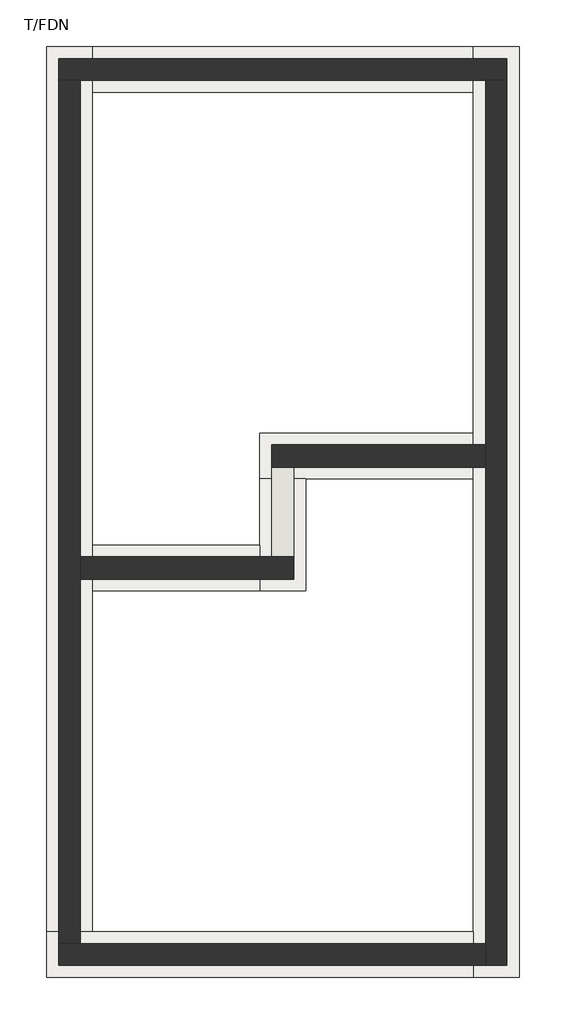
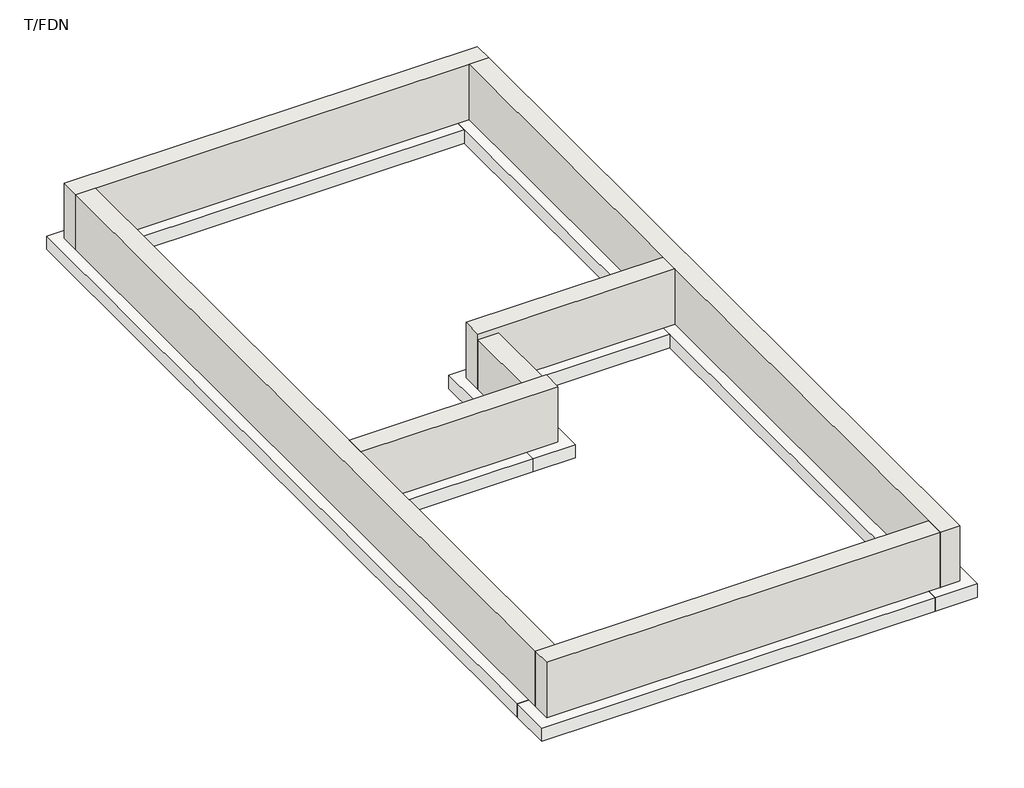
# One storey: 7 footings, 7 walls.
"""IFC4 building model written with IfcOpenShell, lengths in millimetres."""

from ifc_helpers import new_model, si_unit, frame, origin, place, context, project, spatial, polyline, outline, extrude, faceted_brep, element, save

model = new_model("IFC4")

# Units and contexts
model_context = context("Model", 3, world=origin())
ifc_project = project(units=[si_unit("LENGTHUNIT", "METRE", prefix="MILLI")], contexts=[model_context])

# Site, building, storey
site = spatial("IfcSite", under=ifc_project)
building = spatial("IfcBuilding", under=site)
storey = spatial("IfcBuildingStorey", under=building, Name="T/FDN", Elevation=-1250.0)

# Footings
placement = place(None, origin())
element("IfcFooting", 1, ObjectType="Bearing Footing - 900 x 300", at=placement, inside=storey, context=model_context, shape_type="Brep", body=[
    faceted_brep([(8141.5, 241.5, -1250.0), (8141.5, -658.5, -1250.0), (8141.5, -7350.0, -1250.0), (8141.5, -8250.0, -1250.0), (8141.5, -17141.5, -1250.0), (8141.5, -18041.5, -1250.0), (9041.5, -18041.5, -1250.0), (9041.5, 241.5, -1250.0), (9041.5, 241.5, -1550.0), (9041.5, -18041.5, -1550.0), (8141.5, 241.5, -1550.0), (8141.5, -18041.5, -1550.0), (8141.5, -17141.5, -1550.0), (8141.5, -8250.0, -1550.0), (8141.5, -7350.0, -1550.0), (8141.5, -658.5, -1550.0)], [[[0, 1, 2, 3, 4, 5, 6, 7]], [[8, 7, 6, 9]], [[10, 8, 9, 11, 12, 13, 14, 15]], [[0, 10, 15, 14, 13, 12, 11, 5, 4, 3, 2, 1]], [[6, 5, 11, 9]], [[0, 7, 8, 10]]]),
])
element("IfcFooting", 2, ObjectType="Bearing Footing - 900 x 300", at=placement, inside=storey, context=model_context, shape_type="Brep", body=[
    faceted_brep([(-241.5, -17141.5, -1250.0), (-241.5, -18041.5, -1250.0), (8141.5, -18041.5, -1250.0), (8141.5, -17141.5, -1250.0), (658.5, -17141.5, -1250.0), (-241.5, -18041.5, -1550.0), (8141.5, -18041.5, -1550.0), (-241.5, -17141.5, -1550.0), (658.5, -17141.5, -1550.0), (8141.5, -17141.5, -1550.0)], [[[0, 1, 2, 3, 4]], [[1, 5, 6, 2]], [[5, 7, 8, 9, 6]], [[7, 0, 4, 3, 9, 8]], [[3, 2, 6, 9]], [[1, 0, 7, 5]]]),
])
element("IfcFooting", 3, ObjectType="Bearing Footing - 900 x 300", at=placement, inside=storey, context=model_context, shape_type="Brep", body=[
    faceted_brep([(658.5, 241.5, -1250.0), (-241.5, 241.5, -1250.0), (-241.5, -17141.5, -1250.0), (658.5, -17141.5, -1250.0), (658.5, -10450.0, -1250.0), (658.5, -9550.0, -1250.0), (658.5, -658.5, -1250.0), (-241.5, 241.5, -1550.0), (-241.5, -17141.5, -1550.0), (658.5, 241.5, -1550.0), (658.5, -658.5, -1550.0), (658.5, -9550.0, -1550.0), (658.5, -10450.0, -1550.0), (658.5, -17141.5, -1550.0)], [[[0, 1, 2, 3, 4, 5, 6]], [[1, 7, 8, 2]], [[7, 9, 10, 11, 12, 13, 8]], [[9, 0, 6, 5, 4, 3, 13, 12, 11, 10]], [[3, 2, 8, 13]], [[1, 0, 9, 7]]]),
])
element("IfcFooting", 4, ObjectType="Bearing Footing - 900 x 300", at=placement, inside=storey, context=model_context, shape_type="SweptSolid", body=[
    extrude(outline(polyline([(8141.5, 241.5), (8141.5, -658.5), (658.5, -658.5), (658.5, 241.5), (8141.5, 241.5)])), frame((0.0, 0.0, -1550.0), z_axis=(0.0, 0.0, 1.0), x_axis=(1.0, 0.0, 0.0)), (0.0, 0.0, 1.0), 300.0),
])
element("IfcFooting", 5, ObjectType="Bearing Footing - 900 x 300", at=placement, inside=storey, context=model_context, shape_type="Brep", body=[
    faceted_brep([(8141.5, -7350.0, -1250.0), (3950.0, -7350.0, -1250.0), (3950.0, -8250.0, -1250.0), (4850.0, -8250.0, -1250.0), (8141.5, -8250.0, -1250.0), (8141.5, -8250.0, -1550.0), (3950.0, -8250.0, -1550.0), (4850.0, -8250.0, -1550.0), (8141.5, -7350.0, -1550.0), (3950.0, -7350.0, -1550.0)], [[[0, 1, 2, 3, 4]], [[5, 4, 3, 2, 6, 7]], [[8, 5, 7, 6, 9]], [[0, 8, 9, 1]], [[0, 4, 5, 8]], [[2, 1, 9, 6]]]),
])
element("IfcFooting", 6, ObjectType="Bearing Footing - 900 x 300", at=placement, inside=storey, context=model_context, shape_type="Brep", body=[
    faceted_brep([(3950.0, -10450.0, -1250.0), (4850.0, -10450.0, -1250.0), (4850.0, -8250.0, -1250.0), (3950.0, -8250.0, -1250.0), (3950.0, -9550.0, -1250.0), (3950.0, -10450.0, -1550.0), (3950.0, -8250.0, -1550.0), (3950.0, -9550.0, -1550.0), (4850.0, -10450.0, -1550.0), (4850.0, -8250.0, -1550.0)], [[[0, 1, 2, 3, 4]], [[5, 0, 4, 3, 6, 7]], [[8, 5, 7, 6, 9]], [[1, 8, 9, 2]], [[1, 0, 5, 8]], [[3, 2, 9, 6]]]),
])
element("IfcFooting", 7, ObjectType="Bearing Footing - 900 x 300", at=placement, inside=storey, context=model_context, shape_type="SweptSolid", body=[
    extrude(outline(polyline([(658.5, -10450.0), (658.5, -9550.0), (3950.0, -9550.0), (3950.0, -10450.0), (658.5, -10450.0)])), frame((0.0, 0.0, -1550.0), z_axis=(0.0, 0.0, 1.0), x_axis=(1.0, 0.0, 0.0)), (0.0, 0.0, 1.0), 300.0),
])

# Walls
element("IfcWall", 8, ObjectType="Foundation - Concrete (417mm)", at=placement, inside=storey, context=model_context, shape_type="Brep", body=[
    faceted_brep([(0.0, -417.0, -1250.0), (417.0, -417.0, -1250.0), (8383.0, -417.0, -1250.0), (8800.0, -417.0, -1250.0), (8800.0, -417.0, 0.0), (8383.0, -417.0, 0.0), (417.0, -417.0, 0.0), (0.0, -417.0, 0.0), (0.0, 0.0, -1250.0), (0.0, 0.0, 0.0), (8800.0, 0.0, 0.0), (8800.0, 0.0, -1250.0)], [[[0, 1, 2, 3, 4, 5, 6, 7]], [[8, 9, 10, 11]], [[3, 2, 1, 0, 8, 11]], [[7, 6, 5, 4, 10, 9]], [[4, 3, 11, 10]], [[0, 7, 9, 8]]]),
])
element("IfcWall", 9, ObjectType="Foundation - Concrete (417mm)", at=placement, inside=storey, context=model_context, shape_type="Brep", body=[
    faceted_brep([(8383.0, -417.0, -1250.0), (8383.0, -7582.5, -1250.0), (8383.0, -8017.5, -1250.0), (8383.0, -17383.0, -1250.0), (8383.0, -17800.0, -1250.0), (8383.0, -17800.0, 0.0), (8383.0, -17383.0, 0.0), (8383.0, -8017.5, 0.0), (8383.0, -7582.5, 0.0), (8383.0, -417.0, 0.0), (8800.0, -417.0, -1250.0), (8800.0, -417.0, 0.0), (8800.0, -17800.0, 0.0), (8800.0, -17800.0, -1250.0)], [[[0, 1, 2, 3, 4, 5, 6, 7, 8, 9]], [[10, 11, 12, 13]], [[4, 3, 2, 1, 0, 10, 13]], [[9, 8, 7, 6, 5, 12, 11]], [[0, 9, 11, 10]], [[5, 4, 13, 12]]]),
])
element("IfcWall", 10, ObjectType="Foundation - Concrete (417mm)", at=placement, inside=storey, context=model_context, shape_type="Brep", body=[
    faceted_brep([(8383.0, -17383.0, -1250.0), (417.0, -17383.0, -1250.0), (0.0, -17383.0, -1250.0), (0.0, -17383.0, 0.0), (417.0, -17383.0, 0.0), (8383.0, -17383.0, 0.0), (8383.0, -17800.0, -1250.0), (8383.0, -17800.0, 0.0), (0.0, -17800.0, 0.0), (0.0, -17800.0, -1250.0)], [[[0, 1, 2, 3, 4, 5]], [[6, 7, 8, 9]], [[2, 1, 0, 6, 9]], [[5, 4, 3, 8, 7]], [[0, 5, 7, 6]], [[3, 2, 9, 8]]]),
])
element("IfcWall", 11, ObjectType="Foundation - Concrete (417mm)", at=placement, inside=storey, context=model_context, shape_type="Brep", body=[
    faceted_brep([(417.0, -17383.0, -1250.0), (417.0, -10217.5, -1250.0), (417.0, -9782.5, -1250.0), (417.0, -417.0, -1250.0), (417.0, -417.0, 0.0), (417.0, -9782.5, 0.0), (417.0, -10217.5, 0.0), (417.0, -17383.0, 0.0), (0.0, -17383.0, -1250.0), (0.0, -17383.0, 0.0), (0.0, -417.0, 0.0), (0.0, -417.0, -1250.0)], [[[0, 1, 2, 3, 4, 5, 6, 7]], [[8, 9, 10, 11]], [[3, 2, 1, 0, 8, 11]], [[7, 6, 5, 4, 10, 9]], [[4, 3, 11, 10]], [[0, 7, 9, 8]]]),
])
element("IfcWall", 12, ObjectType="Foundation - Concrete (435mm)", at=placement, inside=storey, context=model_context, shape_type="Brep", body=[
    faceted_brep([(8383.0, -7582.5, -1250.0), (4182.5, -7582.5, -1250.0), (4182.5, -7582.5, 0.0), (8383.0, -7582.5, 0.0), (8383.0, -8017.5, -1250.0), (8383.0, -8017.5, 0.0), (4182.5, -8017.5, 0.0), (4182.5, -8017.5, -127.0), (4182.5, -8017.5, -1250.0), (4617.5, -8017.5, -1250.0)], [[[0, 1, 2, 3]], [[4, 5, 6, 7, 8, 9]], [[1, 0, 4, 9, 8]], [[3, 2, 6, 5]], [[0, 3, 5, 4]], [[2, 1, 8, 7, 6]]]),
])
element("IfcWall", 13, ObjectType="Foundation - Concrete (435mm)", at=placement, inside=storey, context=model_context, shape_type="Brep", body=[
    faceted_brep([(417.0, -10217.5, -1250.0), (4617.5, -10217.5, -1250.0), (4617.5, -10217.5, 0.0), (417.0, -10217.5, 0.0), (417.0, -9782.5, -1250.0), (417.0, -9782.5, 0.0), (4617.5, -9782.5, 0.0), (4617.5, -9782.5, -127.0), (4617.5, -9782.5, -1250.0), (4182.5, -9782.5, -1250.0)], [[[0, 1, 2, 3]], [[4, 5, 6, 7, 8, 9]], [[1, 0, 4, 9, 8]], [[3, 2, 6, 5]], [[0, 3, 5, 4]], [[2, 1, 8, 7, 6]]]),
])
element("IfcWall", 14, ObjectType="Foundation - Concrete (435mm)", at=placement, inside=storey, context=model_context, shape_type="SweptSolid", body=[
    extrude(outline(polyline([(4617.5, -8017.5), (4617.5, -9782.5), (4182.5, -9782.5), (4182.5, -8017.5), (4617.5, -8017.5)])), frame((0.0, 0.0, -1250.0), z_axis=(0.0, 0.0, 1.0), x_axis=(1.0, 0.0, 0.0)), (0.0, 0.0, 1.0), 1123.0),
])

save(model, "model.ifc")

# Revit data of these elements
# Project information
#   Host = "https://niras.dk/projects"
#   Project Issue Date = "Issue Date"
#   Project Status = "Project Status"
#   Client Name = "Owner"
#   Project Address = "Enter address here"
#   Project Name = "Duplex Apartment"
#   Project Number = "0001"
#   Category Description = "Duplex"
#   Category Code = "11-16 21 11"
# Type "Bearing Footing - 900 x 300"
#   Manufacturer = "Manufacturer"
#   AccessibilityPerformance = "AccessibilityPerformance"
#   CodePerformance = "CodePerformance"
#   Color = "Color"
#   Constituents = "Constituents"
#   Features = "Features"
#   Finish = "Finish"
#   Grade = "Grade"
#   Material = "Material"
#   ModelReference = "ModelReference"
#   NominalHeight = "NominalHeight"
#   NominalLength = "NominalLength"
#   NominalWidth = "NominalWidth"
#   ProductionYear = "ProductionYear"
#   Reference = "Reference"
#   Shape = "Shape"
#   Size = "Size"
#   SustainabilityPerformance = "SustainabilityPerformance"
#   WarrantyDescription = "WarrantyDescription"
#   WarrantyDurationLabor = "WarrantyDurationLabor"
#   WarrantyDurationParts = "WarrantyDurationParts"
#   WarrantyGuarantorLabor = "WarrantyGuarantorLabor"
#   WarrantyGuarantorParts = "WarrantyGuarantorParts"
#   ExpectedLife = "ExpectedLife"
#   ReplacementCost = "ReplacementCost"
#   AssetAccountingType = "FIXED"
#   Classification Description = "Shallow Foundations"
#   Classification Code = "23-25 05 17"
#   ModelLabel = "ModelLabel"
# Type "Foundation - Concrete (417mm)"
#   Manufacturer = "Manufacturer"
#   AccessibilityPerformance = "AccessibilityPerformance"
#   CodePerformance = "CodePerformance"
#   Color = "Color"
#   Constituents = "Constituents"
#   Features = "Features"
#   Finish = "Finish"
#   Grade = "Grade"
#   Material = "Material"
#   ModelReference = "ModelReference"
#   NominalHeight = "NominalHeight"
#   NominalLength = "NominalLength"
#   NominalWidth = "NominalWidth"
#   ProductionYear = "ProductionYear"
#   Reference = "Reference"
#   Shape = "Shape"
#   Size = "Size"
#   SustainabilityPerformance = "SustainabilityPerformance"
#   WarrantyDescription = "WarrantyDescription"
#   WarrantyDurationLabor = "WarrantyDurationLabor"
#   WarrantyDurationParts = "WarrantyDurationParts"
#   WarrantyGuarantorLabor = "WarrantyGuarantorLabor"
#   WarrantyGuarantorParts = "WarrantyGuarantorParts"
#   ExpectedLife = "ExpectedLife"
#   ReplacementCost = "ReplacementCost"
#   AssetAccountingType = "FIXED"
#   Classification Description = "Concrete Structural Walls"
#   Classification Code = "23-25 30 24 11"
#   ModelLabel = "ModelLabel"
#   Layers, outside or top first: 0.417 m "Concrete - Cast In Situ" (function 1)
# Type "Foundation - Concrete (435mm)"
#   Manufacturer = "Manufacturer"
#   AccessibilityPerformance = "AccessibilityPerformance"
#   CodePerformance = "CodePerformance"
#   Color = "Color"
#   Constituents = "Constituents"
#   Features = "Features"
#   Finish = "Finish"
#   Grade = "Grade"
#   Material = "Material"
#   ModelReference = "ModelReference"
#   NominalHeight = "NominalHeight"
#   NominalLength = "NominalLength"
#   NominalWidth = "NominalWidth"
#   ProductionYear = "ProductionYear"
#   Reference = "Reference"
#   Shape = "Shape"
#   Size = "Size"
#   SustainabilityPerformance = "SustainabilityPerformance"
#   WarrantyDescription = "WarrantyDescription"
#   WarrantyDurationLabor = "WarrantyDurationLabor"
#   WarrantyDurationParts = "WarrantyDurationParts"
#   WarrantyGuarantorLabor = "WarrantyGuarantorLabor"
#   WarrantyGuarantorParts = "WarrantyGuarantorParts"
#   ExpectedLife = "ExpectedLife"
#   ReplacementCost = "ReplacementCost"
#   AssetAccountingType = "FIXED"
#   Classification Description = "Concrete Structural Walls"
#   Classification Code = "23-25 30 24 11"
#   ModelLabel = "ModelLabel"
#   Layers, outside or top first: 0.435 m "Concrete - Cast In Situ" (function 1)
# Elements 1, 2, 3, 4, 5, 6, 7 (IfcFooting, "Bearing Footing - 900 x 300")
#   InstallationDate = "InstallationDate"
#   SerialNumber = "SerialNumber"
#   WarrantyStartDate = "WarrantyStartDate"
#   BarCode = "BarCode"
#   AssetIdentifier = "AssetIdentifier"
#   TagNumber = "TagNumber"
#   Phase Created = New Construction
#   Materials on its faces: "Concrete - Cast In Situ"
# Element 8 (IfcWall, "Foundation - Concrete (417mm)")
#   InstallationDate = "InstallationDate"
#   SerialNumber = "SerialNumber"
#   WarrantyStartDate = "WarrantyStartDate"
#   BarCode = "BarCode"
#   AssetIdentifier = "AssetIdentifier"
#   TagNumber = "TagNumber"
#   URI = "https://niras.dk/projects/0001/wall_1xS3BCk291UvhgP2dvNq2Q"
#   Top Offset = 0.000 m
#   Base Offset = 0.000 m
#   wall height = 1.250 m
#   Phase Created = New Construction
#   Base Constraint = T/FDN
#   Top Constraint = Level 1
#   Materials on its faces: "Concrete - Cast In Situ"
# Element 9 (IfcWall, "Foundation - Concrete (417mm)")
#   InstallationDate = "InstallationDate"
#   SerialNumber = "SerialNumber"
#   WarrantyStartDate = "WarrantyStartDate"
#   BarCode = "BarCode"
#   AssetIdentifier = "AssetIdentifier"
#   TagNumber = "TagNumber"
#   URI = "https://niras.dk/projects/0001/wall_1xS3BCk291UvhgP2dvNq3D"
#   Top Offset = 0.000 m
#   Base Offset = 0.000 m
#   wall height = 1.250 m
#   Phase Created = New Construction
#   Base Constraint = T/FDN
#   Top Constraint = Level 1
#   Materials on its faces: "Concrete - Cast In Situ"
# Element 10 (IfcWall, "Foundation - Concrete (417mm)")
#   InstallationDate = "InstallationDate"
#   SerialNumber = "SerialNumber"
#   WarrantyStartDate = "WarrantyStartDate"
#   BarCode = "BarCode"
#   AssetIdentifier = "AssetIdentifier"
#   TagNumber = "TagNumber"
#   URI = "https://niras.dk/projects/0001/wall_1xS3BCk291UvhgP2dvNq4l"
#   Top Offset = 0.000 m
#   Base Offset = 0.000 m
#   wall height = 1.250 m
#   Phase Created = New Construction
#   Base Constraint = T/FDN
#   Top Constraint = Level 1
#   Materials on its faces: "Concrete - Cast In Situ"
# Element 11 (IfcWall, "Foundation - Concrete (417mm)")
#   InstallationDate = "InstallationDate"
#   SerialNumber = "SerialNumber"
#   WarrantyStartDate = "WarrantyStartDate"
#   BarCode = "BarCode"
#   AssetIdentifier = "AssetIdentifier"
#   TagNumber = "TagNumber"
#   URI = "https://niras.dk/projects/0001/wall_1xS3BCk291UvhgP2dvNq4V"
#   Top Offset = 0.000 m
#   Base Offset = 0.000 m
#   wall height = 1.250 m
#   Phase Created = New Construction
#   Base Constraint = T/FDN
#   Top Constraint = Level 1
#   Materials on its faces: "Concrete - Cast In Situ"
# Element 12 (IfcWall, "Foundation - Concrete (435mm)")
#   InstallationDate = "InstallationDate"
#   SerialNumber = "SerialNumber"
#   WarrantyStartDate = "WarrantyStartDate"
#   BarCode = "BarCode"
#   AssetIdentifier = "AssetIdentifier"
#   TagNumber = "TagNumber"
#   URI = "https://niras.dk/projects/0001/wall_1xS3BCk291UvhgP2dvNq9K"
#   Top Offset = 0.000 m
#   Base Offset = 0.000 m
#   Unconnected Height = 1.250 m
#   wall height = 1.250 m
#   Phase Created = New Construction
#   Base Constraint = T/FDN
#   Top Constraint = Level 1
#   Materials on its faces: "Concrete - Cast In Situ"
# Element 13 (IfcWall, "Foundation - Concrete (435mm)")
#   InstallationDate = "InstallationDate"
#   SerialNumber = "SerialNumber"
#   WarrantyStartDate = "WarrantyStartDate"
#   BarCode = "BarCode"
#   AssetIdentifier = "AssetIdentifier"
#   TagNumber = "TagNumber"
#   URI = "https://niras.dk/projects/0001/wall_1xS3BCk291UvhgP2dvNqAU"
#   Top Offset = 0.000 m
#   Base Offset = 0.000 m
#   Unconnected Height = 1.250 m
#   wall height = 1.250 m
#   Phase Created = New Construction
#   Base Constraint = T/FDN
#   Top Constraint = Level 1
#   Materials on its faces: "Concrete - Cast In Situ"
# Element 14 (IfcWall, "Foundation - Concrete (435mm)")
#   InstallationDate = "InstallationDate"
#   SerialNumber = "SerialNumber"
#   WarrantyStartDate = "WarrantyStartDate"
#   BarCode = "BarCode"
#   AssetIdentifier = "AssetIdentifier"
#   TagNumber = "TagNumber"
#   URI = "https://niras.dk/projects/0001/wall_1xS3BCk291UvhgP2dvNqB%24"
#   Top Offset = -0.127 m
#   Base Offset = 0.000 m
#   wall height = 1.123 m
#   Phase Created = New Construction
#   Base Constraint = T/FDN
#   Top Constraint = Level 1
#   Materials on its faces: "Concrete - Cast In Situ"
# Materials
#   "Concrete - Cast In Situ": class "Concrete", colour RGB 192 192 192, transparency 0
